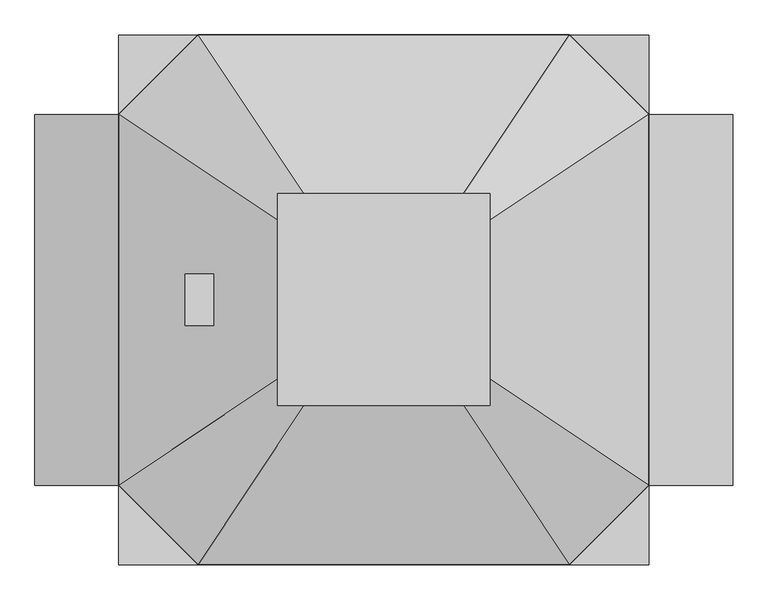
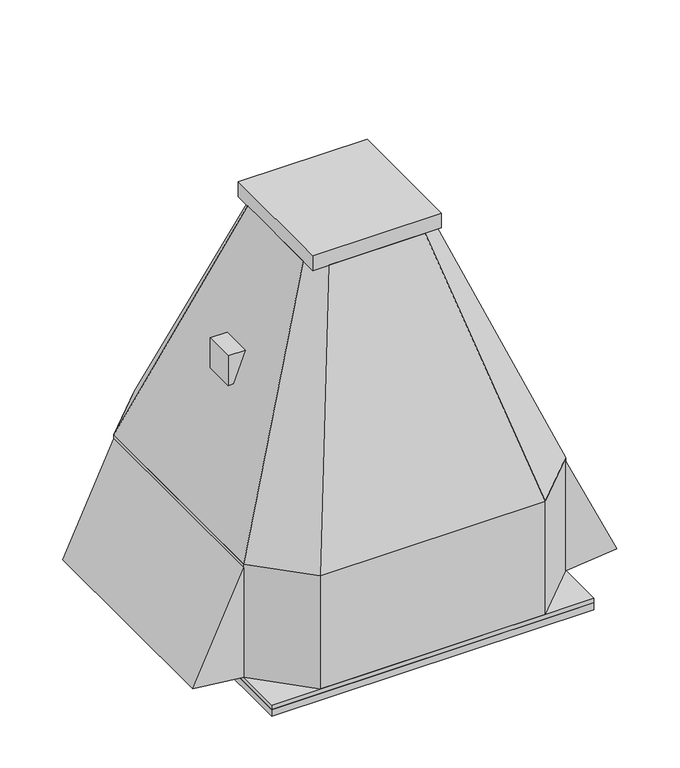
"""IFC4 building model written with IfcOpenShell, lengths in millimetres: proxy geometry, ВЕЗА_Укрос : УКРОС61-056-ДУ600-Н."""

from ifc_helpers import new_model, si_unit, frame, origin, origin_with_axes, place, context, project, spatial, polyline, outline, extrude, faceted_brep, source, transform, mapped, element, save


def mechanical_equipment_0b077342(model_context):
    return source(origin(), model_context, "Body", "SolidModel", [
        faceted_brep([(-164.0, 123.0, 965.0), (-164.0, -123.0, 965.0), (-123.0, -164.0, 965.0), (123.0, -164.0, 965.0), (164.0, -123.0, 965.0), (164.0, 123.0, 965.0), (123.0, 164.0, 965.0), (-123.0, 164.0, 965.0), (-410.0, 287.0, 335.0), (-287.0, 410.0, 335.0), (287.0, 410.0, 335.0), (410.0, 287.0, 335.0), (410.0, -287.0, 335.0), (287.0, -410.0, 335.0), (-287.0, -410.0, 335.0), (-410.0, -287.0, 335.0), (-294.8095238, 40.0, 630.0), (-263.5714286, 40.0, 710.0), (-263.5714286, -40.0, 710.0), (-294.8095238, -40.0, 630.0), (-307.5, 40.0, 630.0), (-307.5, -40.0, 630.0), (-307.5, -40.0, 710.0), (-307.5, 40.0, 710.0)], [[[0, 1, 2, 3, 4, 5, 6, 7]], [[8, 9, 10, 11, 12, 13, 14, 15]], [[1, 0, 8, 15], [16, 17, 18, 19]], [[2, 1, 15, 14]], [[3, 2, 14, 13]], [[4, 3, 13, 12]], [[5, 4, 12, 11]], [[6, 5, 11, 10]], [[7, 6, 10, 9]], [[0, 7, 9, 8]], [[20, 21, 22, 23]], [[20, 23, 17, 16]], [[23, 22, 18, 17]], [[22, 21, 19, 18]], [[21, 20, 16, 19]]]),
        extrude(outline(polyline([(164.0, 164.0), (164.0, -164.0), (-164.0, -164.0), (-164.0, 164.0), (164.0, 164.0)])), frame((0.0, 0.0, 965.0), z_axis=(0.0, 0.0, 1.0), x_axis=(1.0, 0.0, 0.0)), (0.0, 0.0, 1.0), 40.0),
        extrude(outline(polyline([(325.0, -410.0), (44.2169078, -540.0), (30.0, -410.0), (325.0, -410.0)])), frame((0.0, -287.0, 0.0), z_axis=(0.0, 1.0, 0.0), x_axis=(0.0, 0.0, 1.0)), (0.0, 0.0, 1.0), 574.0),
        extrude(outline(polyline([(325.0, 410.0), (30.0, 410.0), (44.2169078, 540.0), (325.0, 410.0)])), frame((0.0, -287.0, 0.0), z_axis=(0.0, 1.0, 0.0), x_axis=(0.0, 0.0, 1.0)), (0.0, 0.0, 1.0), 574.0),
        extrude(outline(polyline([(410.0, 410.0), (410.0, -410.0), (-410.0, -410.0), (-410.0, 410.0), (410.0, 410.0)])), origin_with_axes(), (0.0, 0.0, 1.0), 18.0),
        extrude(outline(polyline([(410.0, 410.0), (410.0, -410.0), (-410.0, -410.0), (-410.0, 410.0), (410.0, 410.0)])), frame((0.0, 0.0, 18.0), z_axis=(0.0, 0.0, 1.0), x_axis=(1.0, 0.0, 0.0)), (0.0, 0.0, 1.0), 12.0),
        extrude(outline(polyline([(-287.0, 410.0), (287.0, 410.0), (410.0, 287.0), (410.0, -287.0), (287.0, -410.0), (-287.0, -410.0), (-410.0, -287.0), (-410.0, 287.0), (-287.0, 410.0)])), frame((0.0, 0.0, 30.0), z_axis=(0.0, 0.0, 1.0), x_axis=(1.0, 0.0, 0.0)), (0.0, 0.0, 1.0), 305.0),
    ])


if __name__ == "__main__":
    model = new_model("IFC4")
    model_context = context("Model", 3, world=origin())
    ifc_project = project(units=[si_unit("LENGTHUNIT", "METRE", prefix="MILLI")], contexts=[model_context])
    site = spatial("IfcSite", under=ifc_project)
    building = spatial("IfcBuilding", under=site)
    placement = place(None, origin())
    mechanical_equipment_shape = mechanical_equipment_0b077342(model_context)
    element("IfcBuildingElementProxy", 1, Name="ВЕЗА_Укрос : УКРОС61-056-ДУ600-Н", ObjectType="ВЕЗА_Укрос : УКРОС61-056-ДУ600-Н", at=placement, inside=building, context=model_context, shape_type="MappedRepresentation", body=[
        mapped(mechanical_equipment_shape, transform((0.0, 0.0, 0.0), x_axis=(1.0, 0.0, 0.0), y_axis=(0.0, 1.0, 0.0), z_axis=(0.0, 0.0, 1.0))),
    ])
    save(model, "model.ifc")

# Revit data of these elements
# Type "ВЕЗА_Укрос : УКРОС61-056-ДУ600-Н"
#   Таблица_размер = "УКРОС-035-063-ДУ-ДУВ"
#   Таблица_масса = "УКРОС-035-063-ДУ_масса_ток"
#   Таблица_марка = "УКРОС-ДУ_035-063_марка_УХЛ"
#   Класс энергоэффективности электродвигателя = "IE2"
#   ВЕЗА_Контакты = "bim@veza.ru"
#   ВЕЗА_Классификатор = "75007"
#   URL = "http://www.veza.ru/upload/iblock/dad/kros2014_24_02_16%20_web.pdf"
#   ADSK_Примечание = ""
#   ADSK_Позиция = "6"
#   ADSK_Наименование краткое = "УКРОС61"
#   ADSK_Наименование = "Вентилятор крышный радиальный дымоудаления УКРОС61; типоразмер 056;режим работы ДУ600; общепромышленный двигатель с номинальной мощностью Nном = 2,20кВт и числом полюсов 4;климатическое исполнение УХЛ1"
#   ADSK_Марка = "УКРОС61-056-ДУ600-Н-00220/4-УХЛ1 ТУ 4861-166-40149153-2013"
#   ADSK_Комплект [instance default] = ""
#   ADSK_Код изделия = ""
#   ADSK_Завод-изготовитель = "ООО \"Веза\", Россия, Москва, ИНН 505001001, info@veza.ru"
#   ADSK_Единица измерения = "шт."
#   ADSK_Дата изменения = "28.02.2020"
#   ADSK_Группирование = ""
#   ADSK_Версия семейства = "Версия 4"
#   ADSK_Версия Revit = "Revit2017"
#   расстояние до виброопор = 250 mm
#   Угол поворота УГО 3D [instance default] = 0°
#   Default Elevation = 1219.2 mm
#   Длина виброопоры [instance default] = 820 mm
#   h_уго_2 = 285 mm
#   h_уго = 335 mm
#   b = 670 mm
#   D1 = 0 mm
#   D = 30 mm
#   C2 = 574 mm
#   C1 = 697 mm
#   B1 = 820 mm
#   H = 1005 mm
#   ADSK_Ток = 5.1 A
#   ADSK_Расход воздуха [instance default] = 0 m³/h
#   ADSK_Размер_Ширина [instance default] = 560 mm
#   ADSK_Размер_Диаметр = 560 mm
#   ADSK_Потеря давления воздуха [instance default] = 0.0 Pa
#   ADSK_Полная мощность = 2315.79 VA
#   ADSK_Номинальная мощность = 2200 W
#   ADSK_Напряжение = 400 V
#   ADSK_Масса = 173
#   ADSK_Коэффициент мощности = 0.95
#   ADSK_Количество = 1
#   B2 = 1080 mm
#   Число полюсов = 4
#   Типоразмер_СТАМ [instance default] = 56
#   Типоразмер = 56
#   Тип вентилятора = 61
#   Режим работы ДУ = 400
#   Масштаб УГО [instance default] = 100
#   Исполнение = 1
#   Видимость патрубка = no
#   Видимость опоры маленьких вентиляторов = yes
#   Видимость виброопоры = no
#   ВЕЗА_Типоразмер = 56
#   ADSK_Частота вращения двигателя = 1500
#   ADSK_Частота вращения вентилятора = 1500
#   ADSK_Количество фаз числовое = 3
#   ADSK_Количество фаз = 3
#   ADSK_Материал = none
#   Использовать масштаб аннотаций [instance default] = (empty)
#   Manufacturer = ""
#   Model = ""
